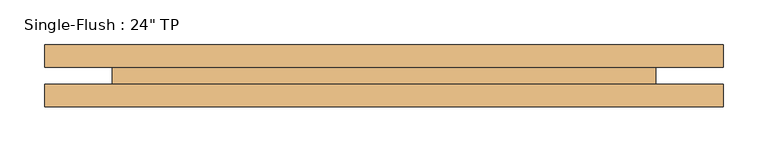
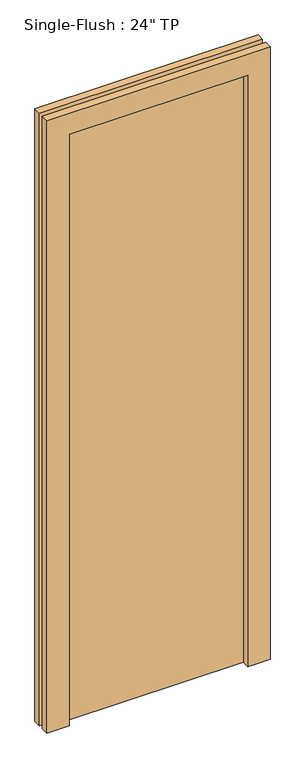
"""IFC4 building model written with IfcOpenShell, lengths in millimetres: door geometry."""

from ifc_helpers import new_model, si_unit, frame, origin, origin_with_axes, place, context, project, spatial, polyline, outline, extrude, source, transform, mapped, element, save


def door_af99bf0a(model_context):
    return source(origin(), model_context, "Body", "SweptSolid", [
        extrude(outline(polyline([(2209.8, -381.0), (0.0, -381.0), (0.0, -304.8), (2133.6, -304.8), (2133.6, 304.8), (0.0, 304.8), (0.0, 381.0), (2209.8, 381.0), (2209.8, -381.0)])), frame((0.0, 9.525, 0.0), z_axis=(0.0, 1.0, 0.0), x_axis=(0.0, 0.0, 1.0)), (0.0, 0.0, 1.0), 25.4),
        extrude(outline(polyline([(2209.8, 381.0), (2209.8, -381.0), (0.0, -381.0), (0.0, -304.8), (2133.6, -304.8), (2133.6, 304.8), (0.0, 304.8), (0.0, 381.0), (2209.8, 381.0)])), frame((0.0, -34.925, 0.0), z_axis=(0.0, 1.0, 0.0), x_axis=(0.0, 0.0, 1.0)), (0.0, 0.0, 1.0), 25.4),
        extrude(outline(polyline([(304.8, -9.525), (-304.8, -9.525), (-304.8, 9.525), (304.8, 9.525), (304.8, -9.525)])), origin_with_axes(), (0.0, 0.0, 1.0), 2133.6),
    ])


if __name__ == "__main__":
    model = new_model("IFC4")
    model_context = context("Model", 3, world=origin())
    ifc_project = project(units=[si_unit("LENGTHUNIT", "METRE", prefix="MILLI")], contexts=[model_context])
    site = spatial("IfcSite", under=ifc_project)
    building = spatial("IfcBuilding", under=site)
    placement = place(None, origin())
    door_shape = door_af99bf0a(model_context)
    element("IfcDoor", 1, ObjectType="Single-Flush : 24\" TP", at=placement, inside=building, context=model_context, shape_type="MappedRepresentation", body=[
        mapped(door_shape, transform((0.0, 0.0, 0.0), x_axis=(1.0, 0.0, 0.0), y_axis=(0.0, 1.0, 0.0), z_axis=(0.0, 0.0, 1.0))),
    ])
    save(model, "model.ifc")

# Revit data of these elements
# Type "Single-Flush : 24\" TP"
#   Type Mark = "59"
#   Construction Type Id = "MDOOR"
#   Assembly Code = "C1020"
#   Analytic Construction = "Metal"
#   Thickness = 0' - 0 3/4"
#   Heat Transfer Coefficient (U) = 3.7021 W/(m²·K)
#   Height = 7' - 0"
#   Trim Projection Ext = 0' - 1"
#   Trim Projection Int = 0' - 1"
#   Trim Width = 0' - 3"
#   Width = 2' - 0"
#   Door Material = Door - Panel
#   Frame Material = Door - Frame
#   Visual Light Transmittance = 0
#   Solar Heat Gain Coefficient = 0
#   Function = (empty or 0)
#   Wall Closure = (empty or 0)
# Element 1 (IfcDoor, "Single-Flush : 24\" TP")
#   Materials on its faces: "Door - Frame", "Door - Panel"
# Materials
#   "Door - Panel": class "Wood", colour RGB 210 159 95, transparency 0
#   "Door - Frame": class "Miscellaneous", colour RGB 118 70 51, transparency 0
